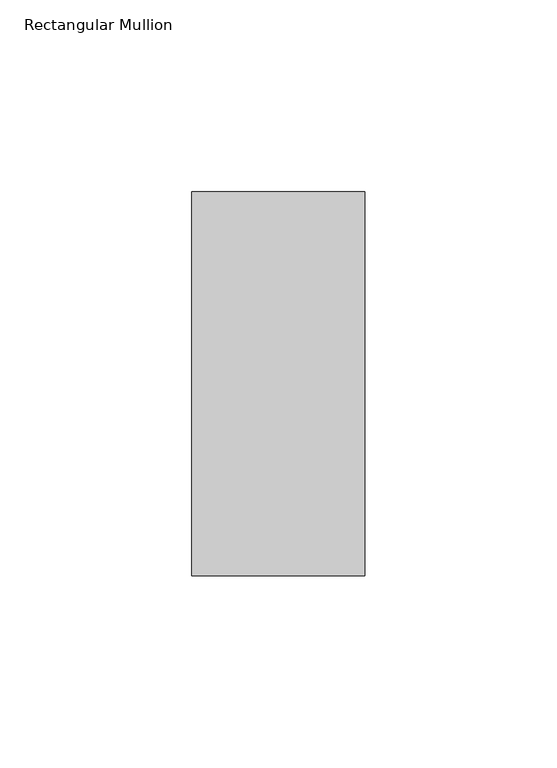
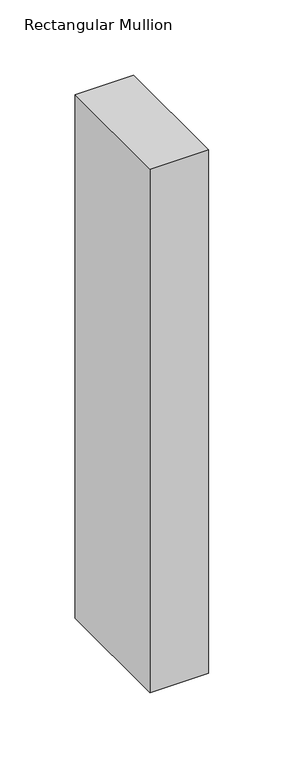
"""IFC4 building model written with IfcOpenShell, lengths in millimetres: member geometry, Rectangular Mullion : 알루미늄_Rectangular Cap_100 x 45."""

import ifcopenshell
import ifcopenshell.guid

model = None  # the IFC model being written
_history = None  # IfcOwnerHistory: only IFC2X3 demands one
_inside = {}  # id of a spatial element -> (the spatial element, [elements in it])
_under = {}  # id of a project, library or spatial element -> (it, [spatial elements below it])
_declared = {}  # id of a project -> (the project, [libraries it declares])
_typed = {}  # id of a type object -> (the type object, [elements of that type])
_made_of = {}  # id of a material, layer set ... -> (it, [elements and type objects made of it])


def new_model(schema):
    """Start an empty IFC model of exactly this schema.

    Asked for "IFC4X3", IfcOpenShell would pick the latest addendum, in which some entities
    have other attributes; the version numbers below select the first issue.
    IFC2X3 requires an IfcOwnerHistory on every rooted entity: one is made here for all.
    """
    global model, _history
    if schema == "IFC4X3":
        model = ifcopenshell.file(schema_version=(4, 3, 0, 0))
    else:
        model = ifcopenshell.file(schema=schema)
    _inside.clear()
    _under.clear()
    _declared.clear()
    _typed.clear()
    _made_of.clear()
    _history = None
    if model.schema == "IFC2X3":
        org = make("IfcOrganization", Name="unknown")
        user = make(
            "IfcPersonAndOrganization",
            ThePerson=make("IfcPerson", FamilyName="unknown"),
            TheOrganization=org,
        )
        app = make(
            "IfcApplication",
            ApplicationDeveloper=org,
            Version="unknown",
            ApplicationFullName="unknown",
            ApplicationIdentifier="unknown",
        )
        _history = make(
            "IfcOwnerHistory",
            OwningUser=user,
            OwningApplication=app,
            ChangeAction="ADDED",
            CreationDate=0,
        )
    return model


def make(cls, **values):
    """One entity of the class cls with the attributes given. An attribute that is None is left unset."""
    return model.create_entity(
        cls, **{name: value for name, value in values.items() if value is not None}
    )


def rooted(cls, **values):
    """An entity with a GlobalId (a new one), such as an element, a storey or a relation."""
    return make(cls, GlobalId=ifcopenshell.guid.new(), OwnerHistory=_history, **values)


def si_unit(unit_type, name, prefix=None):
    """IfcSIUnit, for example si_unit("LENGTHUNIT", "METRE", prefix="MILLI")."""
    return make("IfcSIUnit", UnitType=unit_type, Prefix=prefix, Name=name)


def assignment(units):
    """IfcUnitAssignment: the units of a project."""
    return None if units is None else make("IfcUnitAssignment", Units=units)


def point(xyz):
    """IfcCartesianPoint."""
    return None if xyz is None else make("IfcCartesianPoint", Coordinates=xyz)


def direction(xyz):
    """IfcDirection."""
    return None if xyz is None else make("IfcDirection", DirectionRatios=xyz)


def frame(location, z_axis=None, x_axis=None):
    """IfcAxis2Placement3D, a coordinate frame: its origin and axes. An axis left out is left unset."""
    return make(
        "IfcAxis2Placement3D",
        Location=point(location),
        Axis=direction(z_axis),
        RefDirection=direction(x_axis),
    )


def origin():
    """The frame at (0, 0, 0) with its axes left unset."""
    return frame((0.0, 0.0, 0.0))


def place(relative_to, where):
    """IfcLocalPlacement: puts the frame where relative to a parent placement (None: the world)."""
    return make(
        "IfcLocalPlacement", PlacementRelTo=relative_to, RelativePlacement=where
    )


def context(
    kind, dimensions, precision=None, world=None, true_north=None, identifier=None
):
    """IfcGeometricRepresentationContext, for example the 3D "Model" context."""
    return make(
        "IfcGeometricRepresentationContext",
        ContextIdentifier=identifier,
        ContextType=kind,
        CoordinateSpaceDimension=dimensions,
        Precision=precision,
        WorldCoordinateSystem=world,
        TrueNorth=true_north,
    )


def project(units=None, contexts=None):
    """IfcProject with its units and contexts."""
    return rooted(
        "IfcProject",
        Name="project",
        RepresentationContexts=contexts,
        UnitsInContext=assignment(units),
    )


def spatial(cls, under=None, at=None, **own):
    """A site, building, storey or space (cls), placed at a placement, below another one or the project."""
    s = rooted(cls, ObjectPlacement=at, **own)
    if under is not None:
        _under.setdefault(under.id(), (under, []))[1].append(s)
    return s


def polyline(points):
    """IfcPolyline through the points."""
    return make("IfcPolyline", Points=[point(p) for p in points])


def outline(outer, holes=None, kind="AREA"):
    """IfcArbitraryClosedProfileDef: a profile drawn as a closed curve; with holes, ...WithVoids."""
    if holes is None:
        return make("IfcArbitraryClosedProfileDef", ProfileType=kind, OuterCurve=outer)
    return make(
        "IfcArbitraryProfileDefWithVoids",
        ProfileType=kind,
        OuterCurve=outer,
        InnerCurves=holes,
    )


def extrude(swept, where, along, depth):
    """IfcExtrudedAreaSolid: the profile swept, set in the frame where, extruded along a direction by depth."""
    return make(
        "IfcExtrudedAreaSolid",
        SweptArea=swept,
        Position=where,
        ExtrudedDirection=direction(along),
        Depth=depth,
    )


def shape(context_of_items, identifier, shape_type, items):
    """IfcShapeRepresentation: the items that make up one representation, for example the "Body"."""
    return make(
        "IfcShapeRepresentation",
        ContextOfItems=context_of_items,
        RepresentationIdentifier=identifier,
        RepresentationType=shape_type,
        Items=items,
    )


def source(mapping_origin, context_of_items, identifier, shape_type, items):
    """IfcRepresentationMap: a shape defined once, which mapped items show again and again."""
    return make(
        "IfcRepresentationMap",
        MappingOrigin=mapping_origin,
        MappedRepresentation=shape(context_of_items, identifier, shape_type, items),
    )


def transform(
    local_origin,
    x_axis=None,
    y_axis=None,
    z_axis=None,
    scale=None,
    scale2=None,
    scale3=None,
    uniform=True,
):
    """IfcCartesianTransformationOperator3D, or its non-uniform kind. x_axis, y_axis, z_axis: its Axis1, 2, 3."""
    if uniform:
        return make(
            "IfcCartesianTransformationOperator3D",
            Axis1=direction(x_axis),
            Axis2=direction(y_axis),
            LocalOrigin=point(local_origin),
            Scale=scale,
            Axis3=direction(z_axis),
        )
    return make(
        "IfcCartesianTransformationOperator3DnonUniform",
        Axis1=direction(x_axis),
        Axis2=direction(y_axis),
        LocalOrigin=point(local_origin),
        Scale=scale,
        Axis3=direction(z_axis),
        Scale2=scale2,
        Scale3=scale3,
    )


def mapped(mapping_source, mapping_target):
    """IfcMappedItem: shows the shape of a source again, moved by a transform."""
    return make(
        "IfcMappedItem", MappingSource=mapping_source, MappingTarget=mapping_target
    )


def made_of(thing, what):
    """Note that an element or type object is made of a material, layer set ...; save() writes the relation."""
    if what is not None:
        _made_of.setdefault(what.id(), (what, []))[1].append(thing)
    return thing


def element(
    cls,
    number,
    at=None,
    inside=None,
    cuts=None,
    type_object=None,
    material=None,
    context=None,
    identifier="Body",
    shape_type=None,
    held_by="IfcProductDefinitionShape",
    body=None,
    shapes=None,
    **own,
):
    """One element of the class cls, such as IfcWall. Its Tag is "e" and its number.

    at: its placement. inside: the storey or other place that contains it. cuts: it is an
    opening in that element (IfcRelVoidsElement). A single representation is given by context,
    identifier, shape_type and body (its items); several are given by shapes. held_by: the class
    of the entity that holds the representations. save() writes the other relations.
    """
    e = rooted(cls, Tag="e%d" % number, ObjectPlacement=at, **own)
    if body is not None:
        shapes = [shape(context, identifier, shape_type, body)]
    if shapes is not None:
        e.Representation = make(held_by, Representations=shapes)
    if inside is not None:
        _inside.setdefault(inside.id(), (inside, []))[1].append(e)
    if cuts is not None:
        rooted(
            "IfcRelVoidsElement", RelatingBuildingElement=cuts, RelatedOpeningElement=e
        )
    if type_object is not None:
        _typed.setdefault(type_object.id(), (type_object, []))[1].append(e)
    return made_of(e, material)


def aggregate(whole, parts):
    """IfcRelAggregates: a whole, such as a stair, and the parts it consists of."""
    return rooted("IfcRelAggregates", RelatingObject=whole, RelatedObjects=parts)


def save(model, path):
    """Write the relations noted so far, then the file.

    IfcRelAggregates (storeys below a building ...), IfcRelContainedInSpatialStructure (elements
    in a storey), IfcRelDefinesByType, IfcRelAssociatesMaterial and IfcRelDeclares: one each for
    every whole, place, type object, material and project.
    """
    for whole, parts in _under.values():
        aggregate(whole, parts)
    for where, things in _inside.values():
        rooted(
            "IfcRelContainedInSpatialStructure",
            RelatedElements=things,
            RelatingStructure=where,
        )
    for kind, things in _typed.values():
        rooted("IfcRelDefinesByType", RelatedObjects=things, RelatingType=kind)
    for what, things in _made_of.values():
        rooted("IfcRelAssociatesMaterial", RelatedObjects=things, RelatingMaterial=what)
    for by, libraries in _declared.values():
        rooted("IfcRelDeclares", RelatingContext=by, RelatedDefinitions=libraries)
    model.write(path)


def rectangular_mullion_4dad3324(model_context):
    return source(origin(), model_context, "Body", "SweptSolid", [
        extrude(outline(polyline([(0.0, 50.0), (0.0, -50.0), (-45.0, -50.0), (-45.0, 50.0), (0.0, 50.0)])), frame((0.0, 0.0, -425.0), z_axis=(0.0, 0.0, 1.0), x_axis=(1.0, 0.0, 0.0)), (0.0, 0.0, 1.0), 425.0),
    ])


if __name__ == "__main__":
    model = new_model("IFC4")
    model_context = context("Model", 3, world=origin())
    ifc_project = project(units=[si_unit("LENGTHUNIT", "METRE", prefix="MILLI")], contexts=[model_context])
    site = spatial("IfcSite", under=ifc_project)
    building = spatial("IfcBuilding", under=site)
    placement = place(None, origin())
    rectangular_mullion_shape = rectangular_mullion_4dad3324(model_context)
    element("IfcMember", 1, ObjectType="Rectangular Mullion : 알루미늄_Rectangular Cap_100 x 45", at=placement, inside=building, context=model_context, shape_type="MappedRepresentation", body=[
        mapped(rectangular_mullion_shape, transform((0.0, 0.0, 0.0), x_axis=(1.0, 0.0, 0.0), y_axis=(0.0, 1.0, 0.0), z_axis=(0.0, 0.0, 1.0))),
    ])
    save(model, "model.ifc")

# Revit data of these elements
# Type "Rectangular Mullion : 알루미늄_Rectangular Cap_100 x 45"
#   built-in parameter 1007304 = 0.328084 (stored number, unit not read)
#   built-in parameter 1007301 = 0.0738189 (stored number, unit not read)
#   built-in parameter 1007300 = 0.0738189 (stored number, unit not read)
# Element 1 (IfcMember, "Rectangular Mullion : 알루미늄_Rectangular Cap_100 x 45")
#   Materials on its faces: "00_Metal_Stainless Steel"
# Materials
#   "00_Metal_Stainless Steel": class "Metal", colour RGB 148 148 148, transparency 0, Description = "Steel", Cost = 0
